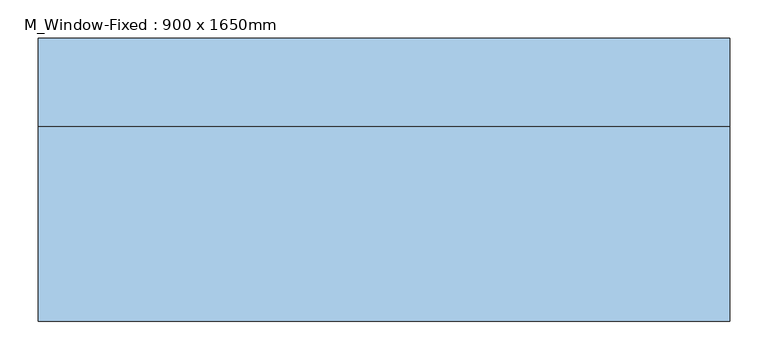
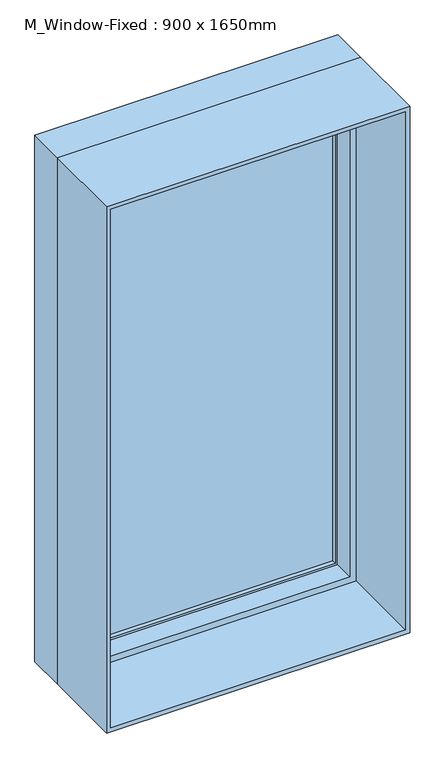
"""IFC4 building model written with IfcOpenShell, lengths in millimetres: window geometry, M_Window-Fixed : 900 x 1650mm."""

from ifc_helpers import new_model, si_unit, frame, origin, place, context, project, spatial, polyline, outline, extrude, faceted_brep, source, transform, mapped, element, save


def m_window_fixed_900_x_1650mm_30845197(model_context):
    return source(origin(), model_context, "Body", "SolidModel", [
        faceted_brep([(450.0, 79.25, 2550.0), (450.0, 193.55, 2550.0), (-450.0, 193.55, 2550.0), (-450.0, 79.25, 2550.0), (-450.0, 193.55, 900.0), (-450.0, 79.25, 900.0), (450.0, 193.55, 900.0), (450.0, 79.25, 900.0), (418.25, 79.25, 2518.25), (418.25, 79.25, 931.75), (-418.25, 79.25, 931.75), (-418.25, 79.25, 2518.25), (-437.3, 193.55, 2537.3), (-437.3, 193.55, 912.7), (437.3, 193.55, 912.7), (437.3, 193.55, 2537.3), (418.25, 142.75, 2518.25), (-418.25, 142.75, 2518.25), (437.3, 142.75, 2537.3), (-437.3, 142.75, 2537.3), (-418.25, 142.75, 931.75), (-437.3, 142.75, 912.7), (418.25, 142.75, 931.75), (437.3, 142.75, 912.7)], [[[0, 1, 2, 3]], [[3, 2, 4, 5]], [[5, 4, 6, 7]], [[3, 5, 7, 0], [8, 9, 10, 11]], [[7, 6, 1, 0]], [[1, 6, 4, 2], [12, 13, 14, 15]], [[16, 8, 11, 17]], [[15, 18, 19, 12]], [[17, 11, 10, 20]], [[12, 19, 21, 13]], [[20, 10, 9, 22]], [[13, 21, 23, 14]], [[22, 9, 8, 16]], [[18, 23, 21, 19], [17, 20, 22, 16]], [[14, 23, 18, 15]]]),
        extrude(outline(polyline([(2550.0, -450.0), (900.0, -450.0), (900.0, 450.0), (2550.0, 450.0), (2550.0, -450.0)]), holes=[polyline([(2537.3, 437.3), (912.7, 437.3), (912.7, -437.3), (2537.3, -437.3), (2537.3, 437.3)])]), frame((0.0, -174.5, 0.0), z_axis=(0.0, 1.0, 0.0), x_axis=(0.0, 0.0, 1.0)), (0.0, 0.0, 1.0), 253.75),
        extrude(outline(polyline([(912.7, 437.3), (2537.3, 437.3), (2537.3, -437.3), (912.7, -437.3), (912.7, 437.3)]), holes=[polyline([(938.1, -411.9), (2511.9, -411.9), (2511.9, 411.9), (938.1, 411.9), (938.1, -411.9)])]), frame((0.0, 142.75, 0.0), z_axis=(0.0, 1.0, 0.0), x_axis=(0.0, 0.0, 1.0)), (0.0, 0.0, 1.0), 44.45),
        extrude(outline(polyline([(411.9, 174.5), (411.9, 168.15), (-411.9, 168.15), (-411.9, 174.5), (411.9, 174.5)])), frame((0.0, 0.0, 938.1), z_axis=(0.0, 0.0, 1.0), x_axis=(1.0, 0.0, 0.0)), (0.0, 0.0, 1.0), 1573.8),
        extrude(outline(polyline([(-411.9, 155.45), (-411.9, 161.8), (411.9, 161.8), (411.9, 155.45), (-411.9, 155.45)])), frame((0.0, 0.0, 938.1), z_axis=(0.0, 0.0, 1.0), x_axis=(1.0, 0.0, 0.0)), (0.0, 0.0, 1.0), 1573.8),
    ])


if __name__ == "__main__":
    model = new_model("IFC4")
    model_context = context("Model", 3, world=origin())
    ifc_project = project(units=[si_unit("LENGTHUNIT", "METRE", prefix="MILLI")], contexts=[model_context])
    site = spatial("IfcSite", under=ifc_project)
    building = spatial("IfcBuilding", under=site)
    placement = place(None, origin())
    m_window_fixed_900_x_1650mm_shape = m_window_fixed_900_x_1650mm_30845197(model_context)
    element("IfcWindow", 1, ObjectType="M_Window-Fixed : 900 x 1650mm", at=placement, inside=building, context=model_context, shape_type="MappedRepresentation", body=[
        mapped(m_window_fixed_900_x_1650mm_shape, transform((0.0, 0.0, 0.0), x_axis=(1.0, 0.0, 0.0), y_axis=(0.0, 1.0, 0.0), z_axis=(0.0, 0.0, 1.0))),
    ])
    save(model, "model.ifc")

# Revit data of these elements
# Type "M_Window-Fixed : 900 x 1650mm"
#   Type Mark = "38"
#   Fire Rating = "0.5h"
#   Assembly Code = "B2020100"
#   Analytic Construction = "Double glazing - domestic"
#   Window Inset [instance default] = 0 mm
#   Wall Thickness [instance default] = 150 mm
#   Visual Light Transmittance = 0.81
#   Thermal Resistance (R) = 0.319569 (m²·K)/W
#   Solar Heat Gain Coefficient = 0.76
#   Rough Width = 915 mm
#   Rough Height = 1665 mm
#   Interior Wall Closure [instance default] = 54.75 mm
#   Height = 1650 mm
#   Heat Transfer Coefficient (U) = 3.12929 W/(m²·K)
#   Frame Extension [instance default] = 6.35 mm
#   Exterior Wall Closure [instance default] = 31.75 mm
#   Extension Jamb [instance default] = 54.75 mm
#   Default Sill Height = 900 mm
#   Width = 900 mm
#   Muntin Visibility = yes
#   Interior Trim Visibility [instance default] = yes
#   Exterior Trim Visibility [instance default] = yes
#   Extension Jamb Visibility [instance default] = yes
#   Muntin Pattern = M_Muntin Pattern_2x2 : M_Muntin Pattern_2x2
#   Interior Trim Material = Wood - Stained
#   Interior Trim = M_Trim-Window-Interior-Flat : Picture Frame
#   Interior Frame Material = Wood - Stained
#   Glass Panel Material = Glass
#   Exterior Trim Material = Clad - White
#   Exterior Trim = M_Trim-Window-Exterior-Flat : with Sill
#   Exterior Frame Material = Clad - White
#   Wall Closure = (empty or 0)
# Element 1 (IfcWindow, "M_Window-Fixed : 900 x 1650mm")
#   Wall Thickness = 349 mm
#   Extension Jamb = 253.75 mm
#   Materials on its faces: "Wood - Stained", "Glass", "Clad - White"
# Materials
#   "Wood - Stained": class "Wood", colour RGB 173 132 96, transparency 0, Cost = 0
#   "Glass": class "Glass", colour RGB 245 245 243, transparency 1, Description = "Soda Lime Glass", Cost = 0
#   "Clad - White": class "Wood", colour RGB 245 245 243, transparency 0, Cost = 0
